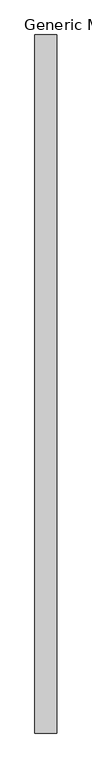
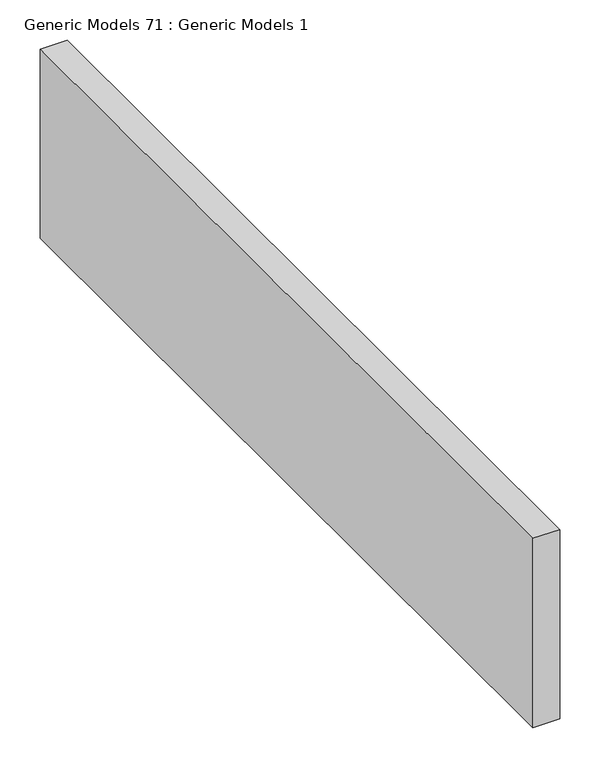
"""IFC4 building model written with IfcOpenShell, lengths in millimetres: proxy geometry, Generic Models 71 : Generic Models 1."""

from ifc_helpers import new_model, si_unit, frame, origin, place, context, project, spatial, polyline, outline, extrude, source, transform, mapped, element, save


def generic_models_71_generic_models_1_508a995f(model_context):
    return source(origin(), model_context, "Body", "SweptSolid", [
        extrude(outline(polyline([(50952.4, 0.0), (50914.3, 0.0), (50914.3, 1219.2), (50952.4, 1219.2), (50952.4, 0.0)])), frame((0.0, 0.0, 5222.478125), z_axis=(0.0, 0.0, 1.0), x_axis=(1.0, 0.0, 0.0)), (0.0, 0.0, 1.0), 285.75),
    ])


if __name__ == "__main__":
    model = new_model("IFC4")
    model_context = context("Model", 3, world=origin())
    ifc_project = project(units=[si_unit("LENGTHUNIT", "METRE", prefix="MILLI")], contexts=[model_context])
    site = spatial("IfcSite", under=ifc_project)
    building = spatial("IfcBuilding", under=site)
    placement = place(None, origin())
    generic_models_71_generic_models_1_shape = generic_models_71_generic_models_1_508a995f(model_context)
    element("IfcBuildingElementProxy", 1, Name="Generic Models 71 : Generic Models 1", ObjectType="Generic Models 71 : Generic Models 1", at=placement, inside=building, context=model_context, shape_type="MappedRepresentation", body=[
        mapped(generic_models_71_generic_models_1_shape, transform((0.0, 0.0, 0.0), x_axis=(1.0, 0.0, 0.0), y_axis=(0.0, 1.0, 0.0), z_axis=(0.0, 0.0, 1.0))),
    ])
    save(model, "model.ifc")

# Revit data of these elements
# Element 1 (IfcBuildingElementProxy, "Generic Models 71 : Generic Models 1")
#   Materials on its faces: "DOUBLE 2X WOOD TOP PLATE"
# Materials
#   "DOUBLE 2X WOOD TOP PLATE": class "Wood", colour RGB 234 198 147, transparency 0, Description = "Pinus Echinata", Cost = 0
